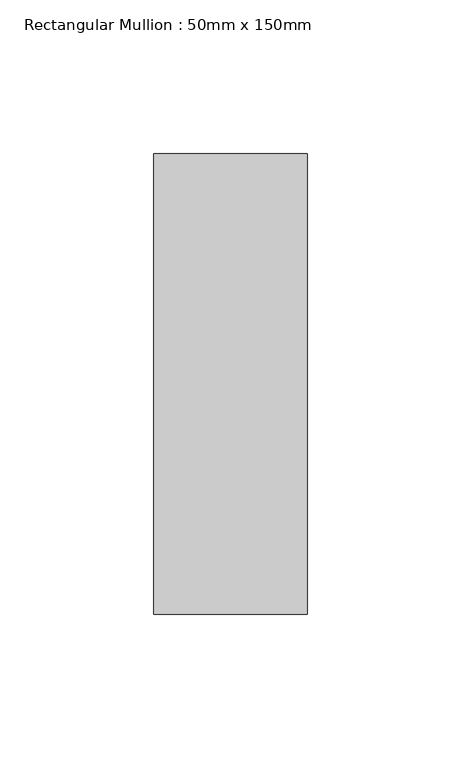
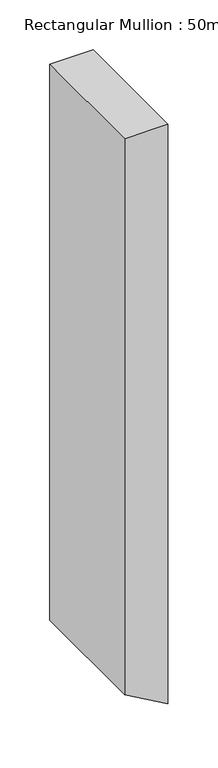
"""IFC4 building model written with IfcOpenShell, lengths in millimetres: member geometry, Rectangular Mullion : 50mm x 150mm."""

import ifcopenshell
import ifcopenshell.guid

model = None  # the IFC model being written
_history = None  # IfcOwnerHistory: only IFC2X3 demands one
_inside = {}  # id of a spatial element -> (the spatial element, [elements in it])
_under = {}  # id of a project, library or spatial element -> (it, [spatial elements below it])
_declared = {}  # id of a project -> (the project, [libraries it declares])
_typed = {}  # id of a type object -> (the type object, [elements of that type])
_made_of = {}  # id of a material, layer set ... -> (it, [elements and type objects made of it])


def new_model(schema):
    """Start an empty IFC model of exactly this schema.

    Asked for "IFC4X3", IfcOpenShell would pick the latest addendum, in which some entities
    have other attributes; the version numbers below select the first issue.
    IFC2X3 requires an IfcOwnerHistory on every rooted entity: one is made here for all.
    """
    global model, _history
    if schema == "IFC4X3":
        model = ifcopenshell.file(schema_version=(4, 3, 0, 0))
    else:
        model = ifcopenshell.file(schema=schema)
    _inside.clear()
    _under.clear()
    _declared.clear()
    _typed.clear()
    _made_of.clear()
    _history = None
    if model.schema == "IFC2X3":
        org = make("IfcOrganization", Name="unknown")
        user = make(
            "IfcPersonAndOrganization",
            ThePerson=make("IfcPerson", FamilyName="unknown"),
            TheOrganization=org,
        )
        app = make(
            "IfcApplication",
            ApplicationDeveloper=org,
            Version="unknown",
            ApplicationFullName="unknown",
            ApplicationIdentifier="unknown",
        )
        _history = make(
            "IfcOwnerHistory",
            OwningUser=user,
            OwningApplication=app,
            ChangeAction="ADDED",
            CreationDate=0,
        )
    return model


def make(cls, **values):
    """One entity of the class cls with the attributes given. An attribute that is None is left unset."""
    return model.create_entity(
        cls, **{name: value for name, value in values.items() if value is not None}
    )


def rooted(cls, **values):
    """An entity with a GlobalId (a new one), such as an element, a storey or a relation."""
    return make(cls, GlobalId=ifcopenshell.guid.new(), OwnerHistory=_history, **values)


def si_unit(unit_type, name, prefix=None):
    """IfcSIUnit, for example si_unit("LENGTHUNIT", "METRE", prefix="MILLI")."""
    return make("IfcSIUnit", UnitType=unit_type, Prefix=prefix, Name=name)


def assignment(units):
    """IfcUnitAssignment: the units of a project."""
    return None if units is None else make("IfcUnitAssignment", Units=units)


def point(xyz):
    """IfcCartesianPoint."""
    return None if xyz is None else make("IfcCartesianPoint", Coordinates=xyz)


def direction(xyz):
    """IfcDirection."""
    return None if xyz is None else make("IfcDirection", DirectionRatios=xyz)


def frame(location, z_axis=None, x_axis=None):
    """IfcAxis2Placement3D, a coordinate frame: its origin and axes. An axis left out is left unset."""
    return make(
        "IfcAxis2Placement3D",
        Location=point(location),
        Axis=direction(z_axis),
        RefDirection=direction(x_axis),
    )


def origin():
    """The frame at (0, 0, 0) with its axes left unset."""
    return frame((0.0, 0.0, 0.0))


def place(relative_to, where):
    """IfcLocalPlacement: puts the frame where relative to a parent placement (None: the world)."""
    return make(
        "IfcLocalPlacement", PlacementRelTo=relative_to, RelativePlacement=where
    )


def context(
    kind, dimensions, precision=None, world=None, true_north=None, identifier=None
):
    """IfcGeometricRepresentationContext, for example the 3D "Model" context."""
    return make(
        "IfcGeometricRepresentationContext",
        ContextIdentifier=identifier,
        ContextType=kind,
        CoordinateSpaceDimension=dimensions,
        Precision=precision,
        WorldCoordinateSystem=world,
        TrueNorth=true_north,
    )


def project(units=None, contexts=None):
    """IfcProject with its units and contexts."""
    return rooted(
        "IfcProject",
        Name="project",
        RepresentationContexts=contexts,
        UnitsInContext=assignment(units),
    )


def spatial(cls, under=None, at=None, **own):
    """A site, building, storey or space (cls), placed at a placement, below another one or the project."""
    s = rooted(cls, ObjectPlacement=at, **own)
    if under is not None:
        _under.setdefault(under.id(), (under, []))[1].append(s)
    return s


def polyline(points):
    """IfcPolyline through the points."""
    return make("IfcPolyline", Points=[point(p) for p in points])


def outline(outer, holes=None, kind="AREA"):
    """IfcArbitraryClosedProfileDef: a profile drawn as a closed curve; with holes, ...WithVoids."""
    if holes is None:
        return make("IfcArbitraryClosedProfileDef", ProfileType=kind, OuterCurve=outer)
    return make(
        "IfcArbitraryProfileDefWithVoids",
        ProfileType=kind,
        OuterCurve=outer,
        InnerCurves=holes,
    )


def extrude(swept, where, along, depth):
    """IfcExtrudedAreaSolid: the profile swept, set in the frame where, extruded along a direction by depth."""
    return make(
        "IfcExtrudedAreaSolid",
        SweptArea=swept,
        Position=where,
        ExtrudedDirection=direction(along),
        Depth=depth,
    )


def shape(context_of_items, identifier, shape_type, items):
    """IfcShapeRepresentation: the items that make up one representation, for example the "Body"."""
    return make(
        "IfcShapeRepresentation",
        ContextOfItems=context_of_items,
        RepresentationIdentifier=identifier,
        RepresentationType=shape_type,
        Items=items,
    )


def source(mapping_origin, context_of_items, identifier, shape_type, items):
    """IfcRepresentationMap: a shape defined once, which mapped items show again and again."""
    return make(
        "IfcRepresentationMap",
        MappingOrigin=mapping_origin,
        MappedRepresentation=shape(context_of_items, identifier, shape_type, items),
    )


def transform(
    local_origin,
    x_axis=None,
    y_axis=None,
    z_axis=None,
    scale=None,
    scale2=None,
    scale3=None,
    uniform=True,
):
    """IfcCartesianTransformationOperator3D, or its non-uniform kind. x_axis, y_axis, z_axis: its Axis1, 2, 3."""
    if uniform:
        return make(
            "IfcCartesianTransformationOperator3D",
            Axis1=direction(x_axis),
            Axis2=direction(y_axis),
            LocalOrigin=point(local_origin),
            Scale=scale,
            Axis3=direction(z_axis),
        )
    return make(
        "IfcCartesianTransformationOperator3DnonUniform",
        Axis1=direction(x_axis),
        Axis2=direction(y_axis),
        LocalOrigin=point(local_origin),
        Scale=scale,
        Axis3=direction(z_axis),
        Scale2=scale2,
        Scale3=scale3,
    )


def mapped(mapping_source, mapping_target):
    """IfcMappedItem: shows the shape of a source again, moved by a transform."""
    return make(
        "IfcMappedItem", MappingSource=mapping_source, MappingTarget=mapping_target
    )


def made_of(thing, what):
    """Note that an element or type object is made of a material, layer set ...; save() writes the relation."""
    if what is not None:
        _made_of.setdefault(what.id(), (what, []))[1].append(thing)
    return thing


def element(
    cls,
    number,
    at=None,
    inside=None,
    cuts=None,
    type_object=None,
    material=None,
    context=None,
    identifier="Body",
    shape_type=None,
    held_by="IfcProductDefinitionShape",
    body=None,
    shapes=None,
    **own,
):
    """One element of the class cls, such as IfcWall. Its Tag is "e" and its number.

    at: its placement. inside: the storey or other place that contains it. cuts: it is an
    opening in that element (IfcRelVoidsElement). A single representation is given by context,
    identifier, shape_type and body (its items); several are given by shapes. held_by: the class
    of the entity that holds the representations. save() writes the other relations.
    """
    e = rooted(cls, Tag="e%d" % number, ObjectPlacement=at, **own)
    if body is not None:
        shapes = [shape(context, identifier, shape_type, body)]
    if shapes is not None:
        e.Representation = make(held_by, Representations=shapes)
    if inside is not None:
        _inside.setdefault(inside.id(), (inside, []))[1].append(e)
    if cuts is not None:
        rooted(
            "IfcRelVoidsElement", RelatingBuildingElement=cuts, RelatedOpeningElement=e
        )
    if type_object is not None:
        _typed.setdefault(type_object.id(), (type_object, []))[1].append(e)
    return made_of(e, material)


def aggregate(whole, parts):
    """IfcRelAggregates: a whole, such as a stair, and the parts it consists of."""
    return rooted("IfcRelAggregates", RelatingObject=whole, RelatedObjects=parts)


def save(model, path):
    """Write the relations noted so far, then the file.

    IfcRelAggregates (storeys below a building ...), IfcRelContainedInSpatialStructure (elements
    in a storey), IfcRelDefinesByType, IfcRelAssociatesMaterial and IfcRelDeclares: one each for
    every whole, place, type object, material and project.
    """
    for whole, parts in _under.values():
        aggregate(whole, parts)
    for where, things in _inside.values():
        rooted(
            "IfcRelContainedInSpatialStructure",
            RelatedElements=things,
            RelatingStructure=where,
        )
    for kind, things in _typed.values():
        rooted("IfcRelDefinesByType", RelatedObjects=things, RelatingType=kind)
    for what, things in _made_of.values():
        rooted("IfcRelAssociatesMaterial", RelatedObjects=things, RelatingMaterial=what)
    for by, libraries in _declared.values():
        rooted("IfcRelDeclares", RelatingContext=by, RelatedDefinitions=libraries)
    model.write(path)


def rectangular_mullion_50mm_x_150mm_c61ed2eb(model_context):
    return source(origin(), model_context, "Body", "SweptSolid", [
        extrude(outline(polyline([(0.0, 0.0), (0.0, -50.0), (-680.4485315, -50.0), (-709.316045, 0.0), (0.0, 0.0)])), frame((0.0, -75.0, 0.0), z_axis=(0.0, 1.0, 0.0), x_axis=(0.0, 0.0, 1.0)), (0.0, 0.0, 1.0), 150.0),
    ])


if __name__ == "__main__":
    model = new_model("IFC4")
    model_context = context("Model", 3, world=origin())
    ifc_project = project(units=[si_unit("LENGTHUNIT", "METRE", prefix="MILLI")], contexts=[model_context])
    site = spatial("IfcSite", under=ifc_project)
    building = spatial("IfcBuilding", under=site)
    placement = place(None, origin())
    rectangular_mullion_50mm_x_150mm_shape = rectangular_mullion_50mm_x_150mm_c61ed2eb(model_context)
    element("IfcMember", 1, ObjectType="Rectangular Mullion : 50mm x 150mm", at=placement, inside=building, context=model_context, shape_type="MappedRepresentation", body=[
        mapped(rectangular_mullion_50mm_x_150mm_shape, transform((0.0, 0.0, 0.0), x_axis=(1.0, 0.0, 0.0), y_axis=(0.0, 1.0, 0.0), z_axis=(0.0, 0.0, 1.0))),
    ])
    save(model, "model.ifc")

# Revit data of these elements
# Type "Rectangular Mullion : 50mm x 150mm"
#   built-in parameter 1007304 = 0.492126 (stored number, unit not read)
#   built-in parameter 1007301 = 0.082021 (stored number, unit not read)
#   built-in parameter 1007300 = 0.082021 (stored number, unit not read)
# Element 1 (IfcMember, "Rectangular Mullion : 50mm x 150mm")
#   Materials on its faces: "Aluminum"
# Materials
#   "Aluminum": class "Metal", colour RGB 247 247 247, transparency 0, Description = "Aluminum 6061", Cost = 0
